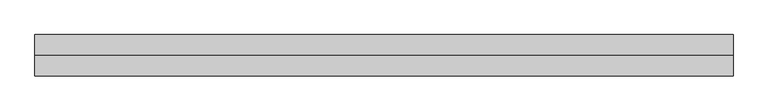
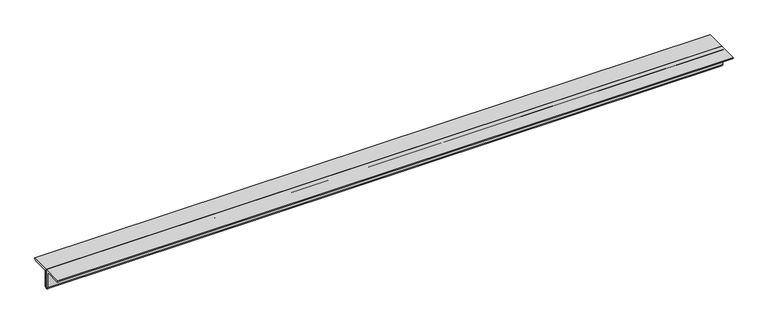
"""IFC4 building model written with IfcOpenShell, lengths in millimetres: member geometry, 0123_Steel Framing_2Ls-KSD3502 : H_SB_AR_S03_2Ls-130x130x12_HBR1."""

from ifc_helpers import new_model, si_unit, point, frame, frame_2d, origin, place, context, project, spatial, polyline, circle_curve, trimmed, segment, composite_curve, outline, extrude, source, transform, mapped, element, save


def member_ee89c48e(model_context):
    return source(origin(), model_context, "Body", "SweptSolid", [
        extrude(outline(composite_curve([segment(polyline([(0.0, 36.4), (0.0, -93.6)]), True, "CONTINUOUS"), segment(trimmed(circle_curve(frame_2d((0.0, -81.6)), 12.0), [point((0.0, -93.6))], [point((-12.0, -81.6))], False, "CARTESIAN"), True, "CONTINUOUS"), segment(polyline([(-12.0, -81.6), (-12.0, 12.4)]), True, "CONTINUOUS"), segment(trimmed(circle_curve(frame_2d((-24.0, 12.4)), 12.0), [point((-12.0, 12.4))], [point((-24.0, 24.4))], True, "CARTESIAN"), True, "CONTINUOUS"), segment(polyline([(-24.0, 24.4), (-118.0, 24.4)]), True, "CONTINUOUS"), segment(trimmed(circle_curve(frame_2d((-118.0, 36.4)), 12.0), [point((-118.0, 24.4))], [point((-130.0, 36.4))], False, "CARTESIAN"), True, "CONTINUOUS"), segment(polyline([(-130.0, 36.4), (0.0, 36.4)]), True, "CONTINUOUS")], self_intersect=False)), frame((-2203.0201459, 0.0, 0.0), z_axis=(1.0, 0.0, 0.0), x_axis=(0.0, 1.0, 0.0)), (0.0, 0.0, 1.0), 4391.0649986),
        extrude(outline(composite_curve([segment(polyline([(0.0, 36.4), (130.0, 36.4)]), True, "CONTINUOUS"), segment(trimmed(circle_curve(frame_2d((118.0, 36.4)), 12.0), [point((130.0, 36.4))], [point((118.0, 24.4))], False, "CARTESIAN"), True, "CONTINUOUS"), segment(polyline([(118.0, 24.4), (24.0, 24.4)]), True, "CONTINUOUS"), segment(trimmed(circle_curve(frame_2d((24.0, 12.4)), 12.0), [point((24.0, 24.4))], [point((12.0, 12.4))], True, "CARTESIAN"), True, "CONTINUOUS"), segment(polyline([(12.0, 12.4), (12.0, -81.6)]), True, "CONTINUOUS"), segment(trimmed(circle_curve(frame_2d((0.0, -81.6)), 12.0), [point((12.0, -81.6))], [point((0.0, -93.6))], False, "CARTESIAN"), True, "CONTINUOUS"), segment(polyline([(0.0, -93.6), (0.0, 36.4)]), True, "CONTINUOUS")], self_intersect=False)), frame((-2203.0201459, 0.0, 0.0), z_axis=(1.0, 0.0, 0.0), x_axis=(0.0, 1.0, 0.0)), (0.0, 0.0, 1.0), 4391.0649986),
    ])


if __name__ == "__main__":
    model = new_model("IFC4")
    model_context = context("Model", 3, world=origin())
    ifc_project = project(units=[si_unit("LENGTHUNIT", "METRE", prefix="MILLI")], contexts=[model_context])
    site = spatial("IfcSite", under=ifc_project)
    building = spatial("IfcBuilding", under=site)
    placement = place(None, origin())
    member_shape = member_ee89c48e(model_context)
    element("IfcMember", 1, ObjectType="0123_Steel Framing_2Ls-KSD3502 : H_SB_AR_S03_2Ls-130x130x12_HBR1", at=placement, inside=building, context=model_context, shape_type="MappedRepresentation", body=[
        mapped(member_shape, transform((0.0, 0.0, 0.0), x_axis=(1.0, 0.0, 0.0), y_axis=(0.0, 1.0, 0.0), z_axis=(0.0, 0.0, 1.0))),
    ])
    save(model, "model.ifc")

# Revit data of these elements
# Type "0123_Steel Framing_2Ls-KSD3502 : H_SB_AR_S03_2Ls-130x130x12_HBR1"
#   Type Mark = "HBR1"
#   Assembly Code = "B10"
#   Legs = "SLBB"
#   W = 8.97
#   Perimeter = 1.04 m²/m
#   Nominal Weight = 46.80 kgf/m
#   Length [instance default] = 1000 mm
#   Space = 0 mm
#   b = 130 mm
#   d = 130 mm
#   t = 12 mm
#   y = 36.4 mm
#   A = 0.005952 m²
#   Structural Material [instance default] = Steel ASTM A36
# Element 1 (IfcMember, "0123_Steel Framing_2Ls-KSD3502 : H_SB_AR_S03_2Ls-130x130x12_HBR1")
#   Materials on its faces: "Steel ASTM A36"
# Materials
#   "Steel ASTM A36": class "Metal", colour RGB 199 199 199, transparency 0, Description = "Structural steel, ASTM A36 Grade B, mill finish", Cost = 0
